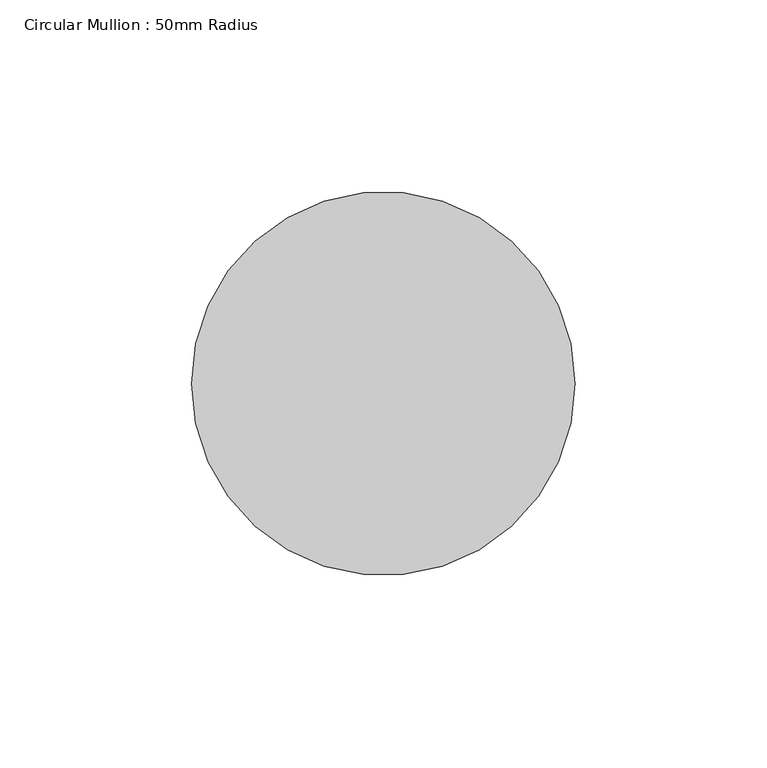
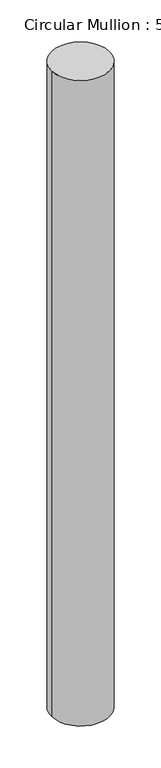
"""IFC4 building model written with IfcOpenShell, lengths in millimetres: member geometry, Circular Mullion : 50mm Radius."""

from ifc_helpers import new_model, si_unit, point, frame, origin, origin_2d, place, context, project, spatial, circle_curve, trimmed, segment, composite_curve, outline, extrude, source, transform, mapped, element, save


def circular_mullion_50mm_radius_3dcaaf55(model_context):
    return source(origin(), model_context, "Body", "SweptSolid", [
        extrude(outline(composite_curve([segment(trimmed(circle_curve(origin_2d(), 50.0), [point((50.0, 0.0))], [point((-50.0, 0.0))], False, "CARTESIAN"), True, "CONTINUOUS"), segment(trimmed(circle_curve(origin_2d(), 50.0), [point((-50.0, 0.0))], [point((50.0, 0.0))], False, "CARTESIAN"), True, "CONTINUOUS")], self_intersect=False)), frame((0.0, 0.0, -1174.8663693), z_axis=(0.0, 0.0, 1.0), x_axis=(1.0, 0.0, 0.0)), (0.0, 0.0, 1.0), 1174.8663693),
    ])


if __name__ == "__main__":
    model = new_model("IFC4")
    model_context = context("Model", 3, world=origin())
    ifc_project = project(units=[si_unit("LENGTHUNIT", "METRE", prefix="MILLI")], contexts=[model_context])
    site = spatial("IfcSite", under=ifc_project)
    building = spatial("IfcBuilding", under=site)
    placement = place(None, origin())
    circular_mullion_50mm_radius_shape = circular_mullion_50mm_radius_3dcaaf55(model_context)
    element("IfcMember", 1, ObjectType="Circular Mullion : 50mm Radius", at=placement, inside=building, context=model_context, shape_type="MappedRepresentation", body=[
        mapped(circular_mullion_50mm_radius_shape, transform((0.0, 0.0, 0.0), x_axis=(1.0, 0.0, 0.0), y_axis=(0.0, 1.0, 0.0), z_axis=(0.0, 0.0, 1.0))),
    ])
    save(model, "model.ifc")

# Revit data of these elements
# Type "Circular Mullion : 50mm Radius"
#   built-in parameter 1007350 = 0.164042 (stored number, unit not read)
# Element 1 (IfcMember, "Circular Mullion : 50mm Radius")
#   Materials on its faces: "Aluminium"
# Materials
#   "Aluminium": class "Metal", colour RGB 247 247 247, transparency 0, Description = "Aluminium 6061", Cost = 0
